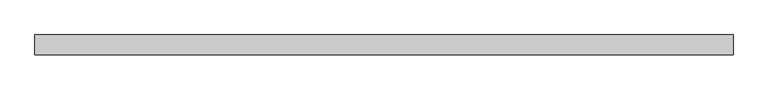
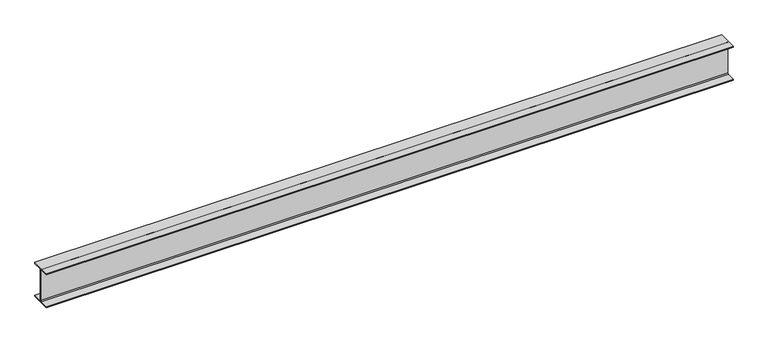
"""IFC4 building model written with IfcOpenShell, lengths in millimetres: beam geometry, Old_Steel Beam_H-KSD3502 : H_SB_ASB_H-350×175x7x11."""

from ifc_helpers import new_model, si_unit, point, frame, frame_2d, origin, place, context, project, spatial, polyline, circle_curve, trimmed, segment, composite_curve, outline, extrude, source, transform, mapped, element, save


def beam_8fb36b93(model_context):
    return source(origin(), model_context, "Body", "SweptSolid", [
        extrude(outline(composite_curve([segment(polyline([(82.5, -141.5), (82.5, -151.7), (-82.5, -151.7), (-82.5, -141.5), (-11.9, -141.5)]), True, "CONTINUOUS"), segment(trimmed(circle_curve(frame_2d((-11.9, -132.6)), 8.9), [point((-11.9, -141.5))], [point((-3.0, -132.6))], True, "CARTESIAN"), True, "CONTINUOUS"), segment(polyline([(-3.0, -132.6), (-3.0, 132.6)]), True, "CONTINUOUS"), segment(trimmed(circle_curve(frame_2d((-11.9, 132.6)), 8.9), [point((-3.0, 132.6))], [point((-11.9, 141.5))], True, "CARTESIAN"), True, "CONTINUOUS"), segment(polyline([(-11.9, 141.5), (-82.5, 141.5), (-82.5, 151.7), (82.5, 151.7), (82.5, 141.5), (11.9, 141.5)]), True, "CONTINUOUS"), segment(trimmed(circle_curve(frame_2d((11.9, 132.6)), 8.9), [point((11.9, 141.5))], [point((3.0, 132.6))], True, "CARTESIAN"), True, "CONTINUOUS"), segment(polyline([(3.0, 132.6), (3.0, -132.6)]), True, "CONTINUOUS"), segment(trimmed(circle_curve(frame_2d((11.9, -132.6)), 8.9), [point((3.0, -132.6))], [point((11.9, -141.5))], True, "CARTESIAN"), True, "CONTINUOUS"), segment(polyline([(11.9, -141.5), (82.5, -141.5)]), True, "CONTINUOUS")], self_intersect=False)), frame((-2769.2350039, 0.0, 0.0), z_axis=(1.0, 0.0, 0.0), x_axis=(0.0, 1.0, 0.0)), (0.0, 0.0, 1.0), 5784.1976903),
    ])


if __name__ == "__main__":
    model = new_model("IFC4")
    model_context = context("Model", 3, world=origin())
    ifc_project = project(units=[si_unit("LENGTHUNIT", "METRE", prefix="MILLI")], contexts=[model_context])
    site = spatial("IfcSite", under=ifc_project)
    building = spatial("IfcBuilding", under=site)
    placement = place(None, origin())
    beam_shape = beam_8fb36b93(model_context)
    element("IfcBeam", 1, ObjectType="Old_Steel Beam_H-KSD3502 : H_SB_ASB_H-350×175x7x11", at=placement, inside=building, context=model_context, shape_type="MappedRepresentation", body=[
        mapped(beam_shape, transform((0.0, 0.0, 0.0), x_axis=(1.0, 0.0, 0.0), y_axis=(0.0, 1.0, 0.0), z_axis=(0.0, 0.0, 1.0))),
    ])
    save(model, "model.ifc")

# Revit data of these elements
# Type "Old_Steel Beam_H-KSD3502 : H_SB_ASB_H-350×175x7x11"
#   Width = 17.5 cm
#   Web Thickness = 0.7 cm
#   Web Fillet = 1.4 cm
#   Warping Constant = 282290.0 cm⁶
#   Torsional Moment of Inertia = 19.4042 cm⁴
#   Torsional Modulus = 1.0 cm³
#   Section Area = 63.14 cm²
#   Plastic Modulus weak axis = 174.0 cm³
#   Plastic Modulus strong axis = 868.0 cm³
#   Perimeter = 1.36 m²/m
#   Nominal Weight = 49.60 kgf/m
#   Moment of Inertia weak axis = 984.00 cm⁴
#   Moment of Inertia strong axis = 13600.00 cm⁴
#   Height = 35.0 cm
#   Flange Thickness = 1.1 cm
#   Elastic Modulus weak axis = 112.0 cm³
#   Elastic Modulus strong axis = 775.0 cm³
#   Centroid Vertical = 17.5 cm
#   Centroid Horizontal = 8.75 cm
#   Length [instance default] = 1.5240 m
#   Structural Material [instance default] = Steel, 45-345
#   Assembly Code = ""
# Element 1 (IfcBeam, "Old_Steel Beam_H-KSD3502 : H_SB_ASB_H-350×175x7x11")
#   Structural Material = none
# Materials
#   "Steel, 45-345": class "Metal", colour RGB 189 187 185, transparency 0, Description = "Steel 345 MPa", Cost = 0
